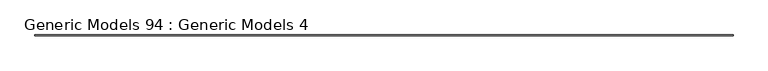
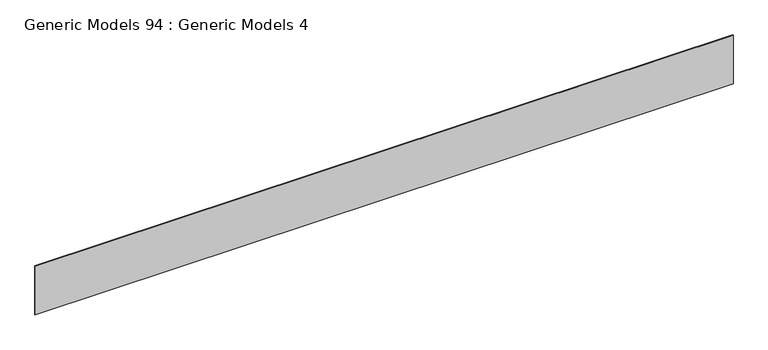
"""IFC4 building model written with IfcOpenShell, lengths in millimetres: proxy geometry, Generic Models 94 : Generic Models 4."""

import ifcopenshell
import ifcopenshell.guid

model = None  # the IFC model being written
_history = None  # IfcOwnerHistory: only IFC2X3 demands one
_inside = {}  # id of a spatial element -> (the spatial element, [elements in it])
_under = {}  # id of a project, library or spatial element -> (it, [spatial elements below it])
_declared = {}  # id of a project -> (the project, [libraries it declares])
_typed = {}  # id of a type object -> (the type object, [elements of that type])
_made_of = {}  # id of a material, layer set ... -> (it, [elements and type objects made of it])


def new_model(schema):
    """Start an empty IFC model of exactly this schema.

    Asked for "IFC4X3", IfcOpenShell would pick the latest addendum, in which some entities
    have other attributes; the version numbers below select the first issue.
    IFC2X3 requires an IfcOwnerHistory on every rooted entity: one is made here for all.
    """
    global model, _history
    if schema == "IFC4X3":
        model = ifcopenshell.file(schema_version=(4, 3, 0, 0))
    else:
        model = ifcopenshell.file(schema=schema)
    _inside.clear()
    _under.clear()
    _declared.clear()
    _typed.clear()
    _made_of.clear()
    _history = None
    if model.schema == "IFC2X3":
        org = make("IfcOrganization", Name="unknown")
        user = make(
            "IfcPersonAndOrganization",
            ThePerson=make("IfcPerson", FamilyName="unknown"),
            TheOrganization=org,
        )
        app = make(
            "IfcApplication",
            ApplicationDeveloper=org,
            Version="unknown",
            ApplicationFullName="unknown",
            ApplicationIdentifier="unknown",
        )
        _history = make(
            "IfcOwnerHistory",
            OwningUser=user,
            OwningApplication=app,
            ChangeAction="ADDED",
            CreationDate=0,
        )
    return model


def make(cls, **values):
    """One entity of the class cls with the attributes given. An attribute that is None is left unset."""
    return model.create_entity(
        cls, **{name: value for name, value in values.items() if value is not None}
    )


def rooted(cls, **values):
    """An entity with a GlobalId (a new one), such as an element, a storey or a relation."""
    return make(cls, GlobalId=ifcopenshell.guid.new(), OwnerHistory=_history, **values)


def si_unit(unit_type, name, prefix=None):
    """IfcSIUnit, for example si_unit("LENGTHUNIT", "METRE", prefix="MILLI")."""
    return make("IfcSIUnit", UnitType=unit_type, Prefix=prefix, Name=name)


def assignment(units):
    """IfcUnitAssignment: the units of a project."""
    return None if units is None else make("IfcUnitAssignment", Units=units)


def point(xyz):
    """IfcCartesianPoint."""
    return None if xyz is None else make("IfcCartesianPoint", Coordinates=xyz)


def direction(xyz):
    """IfcDirection."""
    return None if xyz is None else make("IfcDirection", DirectionRatios=xyz)


def frame(location, z_axis=None, x_axis=None):
    """IfcAxis2Placement3D, a coordinate frame: its origin and axes. An axis left out is left unset."""
    return make(
        "IfcAxis2Placement3D",
        Location=point(location),
        Axis=direction(z_axis),
        RefDirection=direction(x_axis),
    )


def origin():
    """The frame at (0, 0, 0) with its axes left unset."""
    return frame((0.0, 0.0, 0.0))


def place(relative_to, where):
    """IfcLocalPlacement: puts the frame where relative to a parent placement (None: the world)."""
    return make(
        "IfcLocalPlacement", PlacementRelTo=relative_to, RelativePlacement=where
    )


def context(
    kind, dimensions, precision=None, world=None, true_north=None, identifier=None
):
    """IfcGeometricRepresentationContext, for example the 3D "Model" context."""
    return make(
        "IfcGeometricRepresentationContext",
        ContextIdentifier=identifier,
        ContextType=kind,
        CoordinateSpaceDimension=dimensions,
        Precision=precision,
        WorldCoordinateSystem=world,
        TrueNorth=true_north,
    )


def project(units=None, contexts=None):
    """IfcProject with its units and contexts."""
    return rooted(
        "IfcProject",
        Name="project",
        RepresentationContexts=contexts,
        UnitsInContext=assignment(units),
    )


def spatial(cls, under=None, at=None, **own):
    """A site, building, storey or space (cls), placed at a placement, below another one or the project."""
    s = rooted(cls, ObjectPlacement=at, **own)
    if under is not None:
        _under.setdefault(under.id(), (under, []))[1].append(s)
    return s


def polyline(points):
    """IfcPolyline through the points."""
    return make("IfcPolyline", Points=[point(p) for p in points])


def outline(outer, holes=None, kind="AREA"):
    """IfcArbitraryClosedProfileDef: a profile drawn as a closed curve; with holes, ...WithVoids."""
    if holes is None:
        return make("IfcArbitraryClosedProfileDef", ProfileType=kind, OuterCurve=outer)
    return make(
        "IfcArbitraryProfileDefWithVoids",
        ProfileType=kind,
        OuterCurve=outer,
        InnerCurves=holes,
    )


def extrude(swept, where, along, depth):
    """IfcExtrudedAreaSolid: the profile swept, set in the frame where, extruded along a direction by depth."""
    return make(
        "IfcExtrudedAreaSolid",
        SweptArea=swept,
        Position=where,
        ExtrudedDirection=direction(along),
        Depth=depth,
    )


def shape(context_of_items, identifier, shape_type, items):
    """IfcShapeRepresentation: the items that make up one representation, for example the "Body"."""
    return make(
        "IfcShapeRepresentation",
        ContextOfItems=context_of_items,
        RepresentationIdentifier=identifier,
        RepresentationType=shape_type,
        Items=items,
    )


def source(mapping_origin, context_of_items, identifier, shape_type, items):
    """IfcRepresentationMap: a shape defined once, which mapped items show again and again."""
    return make(
        "IfcRepresentationMap",
        MappingOrigin=mapping_origin,
        MappedRepresentation=shape(context_of_items, identifier, shape_type, items),
    )


def transform(
    local_origin,
    x_axis=None,
    y_axis=None,
    z_axis=None,
    scale=None,
    scale2=None,
    scale3=None,
    uniform=True,
):
    """IfcCartesianTransformationOperator3D, or its non-uniform kind. x_axis, y_axis, z_axis: its Axis1, 2, 3."""
    if uniform:
        return make(
            "IfcCartesianTransformationOperator3D",
            Axis1=direction(x_axis),
            Axis2=direction(y_axis),
            LocalOrigin=point(local_origin),
            Scale=scale,
            Axis3=direction(z_axis),
        )
    return make(
        "IfcCartesianTransformationOperator3DnonUniform",
        Axis1=direction(x_axis),
        Axis2=direction(y_axis),
        LocalOrigin=point(local_origin),
        Scale=scale,
        Axis3=direction(z_axis),
        Scale2=scale2,
        Scale3=scale3,
    )


def mapped(mapping_source, mapping_target):
    """IfcMappedItem: shows the shape of a source again, moved by a transform."""
    return make(
        "IfcMappedItem", MappingSource=mapping_source, MappingTarget=mapping_target
    )


def made_of(thing, what):
    """Note that an element or type object is made of a material, layer set ...; save() writes the relation."""
    if what is not None:
        _made_of.setdefault(what.id(), (what, []))[1].append(thing)
    return thing


def element(
    cls,
    number,
    at=None,
    inside=None,
    cuts=None,
    type_object=None,
    material=None,
    context=None,
    identifier="Body",
    shape_type=None,
    held_by="IfcProductDefinitionShape",
    body=None,
    shapes=None,
    **own,
):
    """One element of the class cls, such as IfcWall. Its Tag is "e" and its number.

    at: its placement. inside: the storey or other place that contains it. cuts: it is an
    opening in that element (IfcRelVoidsElement). A single representation is given by context,
    identifier, shape_type and body (its items); several are given by shapes. held_by: the class
    of the entity that holds the representations. save() writes the other relations.
    """
    e = rooted(cls, Tag="e%d" % number, ObjectPlacement=at, **own)
    if body is not None:
        shapes = [shape(context, identifier, shape_type, body)]
    if shapes is not None:
        e.Representation = make(held_by, Representations=shapes)
    if inside is not None:
        _inside.setdefault(inside.id(), (inside, []))[1].append(e)
    if cuts is not None:
        rooted(
            "IfcRelVoidsElement", RelatingBuildingElement=cuts, RelatedOpeningElement=e
        )
    if type_object is not None:
        _typed.setdefault(type_object.id(), (type_object, []))[1].append(e)
    return made_of(e, material)


def aggregate(whole, parts):
    """IfcRelAggregates: a whole, such as a stair, and the parts it consists of."""
    return rooted("IfcRelAggregates", RelatingObject=whole, RelatedObjects=parts)


def save(model, path):
    """Write the relations noted so far, then the file.

    IfcRelAggregates (storeys below a building ...), IfcRelContainedInSpatialStructure (elements
    in a storey), IfcRelDefinesByType, IfcRelAssociatesMaterial and IfcRelDeclares: one each for
    every whole, place, type object, material and project.
    """
    for whole, parts in _under.values():
        aggregate(whole, parts)
    for where, things in _inside.values():
        rooted(
            "IfcRelContainedInSpatialStructure",
            RelatedElements=things,
            RelatingStructure=where,
        )
    for kind, things in _typed.values():
        rooted("IfcRelDefinesByType", RelatedObjects=things, RelatingType=kind)
    for what, things in _made_of.values():
        rooted("IfcRelAssociatesMaterial", RelatedObjects=things, RelatingMaterial=what)
    for by, libraries in _declared.values():
        rooted("IfcRelDeclares", RelatingContext=by, RelatedDefinitions=libraries)
    model.write(path)


def generic_models_94_generic_models_4_2f52971e(model_context):
    return source(origin(), model_context, "Body", "SweptSolid", [
        extrude(outline(polyline([(-2152.1733045, 51452.647716), (-2152.1733045, 51433.597716), (-20795.7733045, 51433.597716), (-20795.7733045, 51452.647716), (-2152.1733045, 51452.647716)])), frame((0.0, 0.0, 125737.7312018), z_axis=(0.0, 0.0, 1.0), x_axis=(1.0, 0.0, 0.0)), (0.0, 0.0, 1.0), 1370.7371642),
    ])


if __name__ == "__main__":
    model = new_model("IFC4")
    model_context = context("Model", 3, world=origin())
    ifc_project = project(units=[si_unit("LENGTHUNIT", "METRE", prefix="MILLI")], contexts=[model_context])
    site = spatial("IfcSite", under=ifc_project)
    building = spatial("IfcBuilding", under=site)
    placement = place(None, origin())
    generic_models_94_generic_models_4_shape = generic_models_94_generic_models_4_2f52971e(model_context)
    element("IfcBuildingElementProxy", 1, Name="Generic Models 94 : Generic Models 4", ObjectType="Generic Models 94 : Generic Models 4", at=placement, inside=building, context=model_context, shape_type="MappedRepresentation", body=[
        mapped(generic_models_94_generic_models_4_shape, transform((0.0, 0.0, 0.0), x_axis=(1.0, 0.0, 0.0), y_axis=(0.0, 1.0, 0.0), z_axis=(0.0, 0.0, 1.0))),
    ])
    save(model, "model.ifc")

# Revit data of these elements
# Element 1 (IfcBuildingElementProxy, "Generic Models 94 : Generic Models 4")
#   Materials on its faces: "_CDX PLYWOOD - SEE STRUCT DWGs"
# Materials
#   "_CDX PLYWOOD - SEE STRUCT DWGs": class "Generic", colour RGB 98 75 74, transparency 0, Cost = 0
